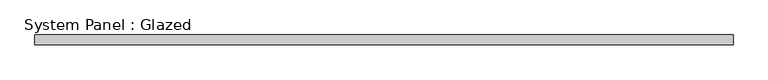
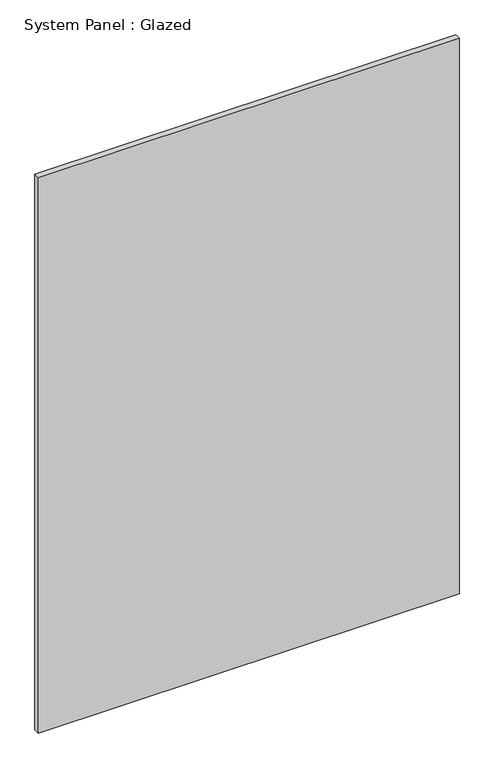
"""IFC4 building model written with IfcOpenShell, lengths in millimetres: plate geometry, System Panel : Glazed."""

import ifcopenshell
import ifcopenshell.guid

model = None  # the IFC model being written
_history = None  # IfcOwnerHistory: only IFC2X3 demands one
_inside = {}  # id of a spatial element -> (the spatial element, [elements in it])
_under = {}  # id of a project, library or spatial element -> (it, [spatial elements below it])
_declared = {}  # id of a project -> (the project, [libraries it declares])
_typed = {}  # id of a type object -> (the type object, [elements of that type])
_made_of = {}  # id of a material, layer set ... -> (it, [elements and type objects made of it])


def new_model(schema):
    """Start an empty IFC model of exactly this schema.

    Asked for "IFC4X3", IfcOpenShell would pick the latest addendum, in which some entities
    have other attributes; the version numbers below select the first issue.
    IFC2X3 requires an IfcOwnerHistory on every rooted entity: one is made here for all.
    """
    global model, _history
    if schema == "IFC4X3":
        model = ifcopenshell.file(schema_version=(4, 3, 0, 0))
    else:
        model = ifcopenshell.file(schema=schema)
    _inside.clear()
    _under.clear()
    _declared.clear()
    _typed.clear()
    _made_of.clear()
    _history = None
    if model.schema == "IFC2X3":
        org = make("IfcOrganization", Name="unknown")
        user = make(
            "IfcPersonAndOrganization",
            ThePerson=make("IfcPerson", FamilyName="unknown"),
            TheOrganization=org,
        )
        app = make(
            "IfcApplication",
            ApplicationDeveloper=org,
            Version="unknown",
            ApplicationFullName="unknown",
            ApplicationIdentifier="unknown",
        )
        _history = make(
            "IfcOwnerHistory",
            OwningUser=user,
            OwningApplication=app,
            ChangeAction="ADDED",
            CreationDate=0,
        )
    return model


def make(cls, **values):
    """One entity of the class cls with the attributes given. An attribute that is None is left unset."""
    return model.create_entity(
        cls, **{name: value for name, value in values.items() if value is not None}
    )


def rooted(cls, **values):
    """An entity with a GlobalId (a new one), such as an element, a storey or a relation."""
    return make(cls, GlobalId=ifcopenshell.guid.new(), OwnerHistory=_history, **values)


def si_unit(unit_type, name, prefix=None):
    """IfcSIUnit, for example si_unit("LENGTHUNIT", "METRE", prefix="MILLI")."""
    return make("IfcSIUnit", UnitType=unit_type, Prefix=prefix, Name=name)


def assignment(units):
    """IfcUnitAssignment: the units of a project."""
    return None if units is None else make("IfcUnitAssignment", Units=units)


def point(xyz):
    """IfcCartesianPoint."""
    return None if xyz is None else make("IfcCartesianPoint", Coordinates=xyz)


def direction(xyz):
    """IfcDirection."""
    return None if xyz is None else make("IfcDirection", DirectionRatios=xyz)


def frame(location, z_axis=None, x_axis=None):
    """IfcAxis2Placement3D, a coordinate frame: its origin and axes. An axis left out is left unset."""
    return make(
        "IfcAxis2Placement3D",
        Location=point(location),
        Axis=direction(z_axis),
        RefDirection=direction(x_axis),
    )


def origin():
    """The frame at (0, 0, 0) with its axes left unset."""
    return frame((0.0, 0.0, 0.0))


def origin_with_axes():
    """The frame at (0, 0, 0) with the z axis (0, 0, 1) and the x axis (1, 0, 0) written out."""
    return frame((0.0, 0.0, 0.0), z_axis=(0.0, 0.0, 1.0), x_axis=(1.0, 0.0, 0.0))


def place(relative_to, where):
    """IfcLocalPlacement: puts the frame where relative to a parent placement (None: the world)."""
    return make(
        "IfcLocalPlacement", PlacementRelTo=relative_to, RelativePlacement=where
    )


def context(
    kind, dimensions, precision=None, world=None, true_north=None, identifier=None
):
    """IfcGeometricRepresentationContext, for example the 3D "Model" context."""
    return make(
        "IfcGeometricRepresentationContext",
        ContextIdentifier=identifier,
        ContextType=kind,
        CoordinateSpaceDimension=dimensions,
        Precision=precision,
        WorldCoordinateSystem=world,
        TrueNorth=true_north,
    )


def project(units=None, contexts=None):
    """IfcProject with its units and contexts."""
    return rooted(
        "IfcProject",
        Name="project",
        RepresentationContexts=contexts,
        UnitsInContext=assignment(units),
    )


def spatial(cls, under=None, at=None, **own):
    """A site, building, storey or space (cls), placed at a placement, below another one or the project."""
    s = rooted(cls, ObjectPlacement=at, **own)
    if under is not None:
        _under.setdefault(under.id(), (under, []))[1].append(s)
    return s


def polyline(points):
    """IfcPolyline through the points."""
    return make("IfcPolyline", Points=[point(p) for p in points])


def outline(outer, holes=None, kind="AREA"):
    """IfcArbitraryClosedProfileDef: a profile drawn as a closed curve; with holes, ...WithVoids."""
    if holes is None:
        return make("IfcArbitraryClosedProfileDef", ProfileType=kind, OuterCurve=outer)
    return make(
        "IfcArbitraryProfileDefWithVoids",
        ProfileType=kind,
        OuterCurve=outer,
        InnerCurves=holes,
    )


def extrude(swept, where, along, depth):
    """IfcExtrudedAreaSolid: the profile swept, set in the frame where, extruded along a direction by depth."""
    return make(
        "IfcExtrudedAreaSolid",
        SweptArea=swept,
        Position=where,
        ExtrudedDirection=direction(along),
        Depth=depth,
    )


def shape(context_of_items, identifier, shape_type, items):
    """IfcShapeRepresentation: the items that make up one representation, for example the "Body"."""
    return make(
        "IfcShapeRepresentation",
        ContextOfItems=context_of_items,
        RepresentationIdentifier=identifier,
        RepresentationType=shape_type,
        Items=items,
    )


def source(mapping_origin, context_of_items, identifier, shape_type, items):
    """IfcRepresentationMap: a shape defined once, which mapped items show again and again."""
    return make(
        "IfcRepresentationMap",
        MappingOrigin=mapping_origin,
        MappedRepresentation=shape(context_of_items, identifier, shape_type, items),
    )


def transform(
    local_origin,
    x_axis=None,
    y_axis=None,
    z_axis=None,
    scale=None,
    scale2=None,
    scale3=None,
    uniform=True,
):
    """IfcCartesianTransformationOperator3D, or its non-uniform kind. x_axis, y_axis, z_axis: its Axis1, 2, 3."""
    if uniform:
        return make(
            "IfcCartesianTransformationOperator3D",
            Axis1=direction(x_axis),
            Axis2=direction(y_axis),
            LocalOrigin=point(local_origin),
            Scale=scale,
            Axis3=direction(z_axis),
        )
    return make(
        "IfcCartesianTransformationOperator3DnonUniform",
        Axis1=direction(x_axis),
        Axis2=direction(y_axis),
        LocalOrigin=point(local_origin),
        Scale=scale,
        Axis3=direction(z_axis),
        Scale2=scale2,
        Scale3=scale3,
    )


def mapped(mapping_source, mapping_target):
    """IfcMappedItem: shows the shape of a source again, moved by a transform."""
    return make(
        "IfcMappedItem", MappingSource=mapping_source, MappingTarget=mapping_target
    )


def made_of(thing, what):
    """Note that an element or type object is made of a material, layer set ...; save() writes the relation."""
    if what is not None:
        _made_of.setdefault(what.id(), (what, []))[1].append(thing)
    return thing


def element(
    cls,
    number,
    at=None,
    inside=None,
    cuts=None,
    type_object=None,
    material=None,
    context=None,
    identifier="Body",
    shape_type=None,
    held_by="IfcProductDefinitionShape",
    body=None,
    shapes=None,
    **own,
):
    """One element of the class cls, such as IfcWall. Its Tag is "e" and its number.

    at: its placement. inside: the storey or other place that contains it. cuts: it is an
    opening in that element (IfcRelVoidsElement). A single representation is given by context,
    identifier, shape_type and body (its items); several are given by shapes. held_by: the class
    of the entity that holds the representations. save() writes the other relations.
    """
    e = rooted(cls, Tag="e%d" % number, ObjectPlacement=at, **own)
    if body is not None:
        shapes = [shape(context, identifier, shape_type, body)]
    if shapes is not None:
        e.Representation = make(held_by, Representations=shapes)
    if inside is not None:
        _inside.setdefault(inside.id(), (inside, []))[1].append(e)
    if cuts is not None:
        rooted(
            "IfcRelVoidsElement", RelatingBuildingElement=cuts, RelatedOpeningElement=e
        )
    if type_object is not None:
        _typed.setdefault(type_object.id(), (type_object, []))[1].append(e)
    return made_of(e, material)


def aggregate(whole, parts):
    """IfcRelAggregates: a whole, such as a stair, and the parts it consists of."""
    return rooted("IfcRelAggregates", RelatingObject=whole, RelatedObjects=parts)


def save(model, path):
    """Write the relations noted so far, then the file.

    IfcRelAggregates (storeys below a building ...), IfcRelContainedInSpatialStructure (elements
    in a storey), IfcRelDefinesByType, IfcRelAssociatesMaterial and IfcRelDeclares: one each for
    every whole, place, type object, material and project.
    """
    for whole, parts in _under.values():
        aggregate(whole, parts)
    for where, things in _inside.values():
        rooted(
            "IfcRelContainedInSpatialStructure",
            RelatedElements=things,
            RelatingStructure=where,
        )
    for kind, things in _typed.values():
        rooted("IfcRelDefinesByType", RelatedObjects=things, RelatingType=kind)
    for what, things in _made_of.values():
        rooted("IfcRelAssociatesMaterial", RelatedObjects=things, RelatingMaterial=what)
    for by, libraries in _declared.values():
        rooted("IfcRelDeclares", RelatingContext=by, RelatedDefinitions=libraries)
    model.write(path)


def system_panel_glazed_9668c591(model_context):
    return source(origin(), model_context, "Body", "SweptSolid", [
        extrude(outline(polyline([(877.5, 24.5), (-877.5, 24.5), (-877.5, 49.5), (877.5, 49.5), (877.5, 24.5)])), origin_with_axes(), (0.0, 0.0, 1.0), 2450.0),
    ])


if __name__ == "__main__":
    model = new_model("IFC4")
    model_context = context("Model", 3, world=origin())
    ifc_project = project(units=[si_unit("LENGTHUNIT", "METRE", prefix="MILLI")], contexts=[model_context])
    site = spatial("IfcSite", under=ifc_project)
    building = spatial("IfcBuilding", under=site)
    placement = place(None, origin())
    system_panel_glazed_shape = system_panel_glazed_9668c591(model_context)
    element("IfcPlate", 1, ObjectType="System Panel : Glazed", at=placement, inside=building, context=model_context, shape_type="MappedRepresentation", body=[
        mapped(system_panel_glazed_shape, transform((0.0, 0.0, 0.0), x_axis=(1.0, 0.0, 0.0), y_axis=(0.0, 1.0, 0.0), z_axis=(0.0, 0.0, 1.0))),
    ])
    save(model, "model.ifc")

# Revit data of these elements
# Type "System Panel : Glazed"
#   Keynote = "H11"
#   Construction Type Id = "GSP4R"
#   Analytic Construction = "1/8 in Pilkington single glazing"
#   Visual Light Transmittance = 0.9
#   Solar Heat Gain Coefficient = 0.86
#   Heat Transfer Coefficient (U) = 6.7069 W/(m²·K)
# Element 1 (IfcPlate, "System Panel : Glazed")
#   Materials on its faces: "Glass"
# Materials
#   "Glass": class "Glass", colour RGB 0 128 192, transparency 0.9, Description = "Soda Lime Glass", Cost = 0
